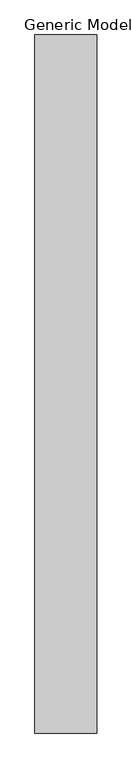
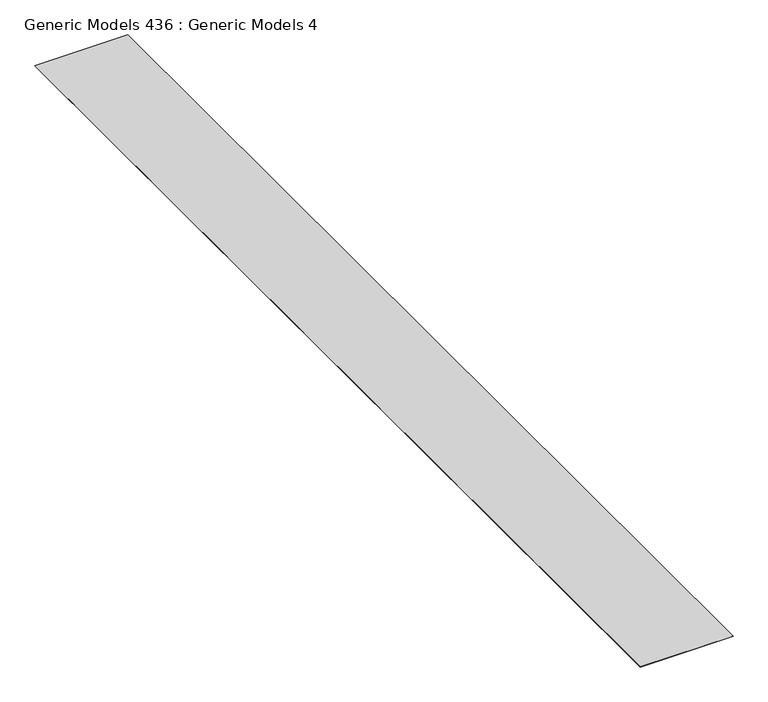
"""IFC4 building model written with IfcOpenShell, lengths in millimetres: proxy geometry, Generic Models 436 : Generic Models 4."""

from ifc_helpers import new_model, si_unit, frame, origin, place, context, project, spatial, polyline, outline, extrude, source, transform, mapped, element, save


def generic_models_436_generic_models_4_e7a1f224(model_context):
    return source(origin(), model_context, "Body", "SweptSolid", [
        extrude(outline(polyline([(9684.9758543, -5493.3230338), (8572.3263705, -5493.3230338), (8572.3263705, 7054.2769662), (9684.9758543, 7054.2769662), (9684.9758543, -5493.3230338)])), frame((0.0, 0.0, 123244.2139347), z_axis=(0.0, 0.0, 1.0), x_axis=(1.0, 0.0, 0.0)), (0.0, 0.0, 1.0), 1.5875),
    ])


if __name__ == "__main__":
    model = new_model("IFC4")
    model_context = context("Model", 3, world=origin())
    ifc_project = project(units=[si_unit("LENGTHUNIT", "METRE", prefix="MILLI")], contexts=[model_context])
    site = spatial("IfcSite", under=ifc_project)
    building = spatial("IfcBuilding", under=site)
    placement = place(None, origin())
    generic_models_436_generic_models_4_shape = generic_models_436_generic_models_4_e7a1f224(model_context)
    element("IfcBuildingElementProxy", 1, Name="Generic Models 436 : Generic Models 4", ObjectType="Generic Models 436 : Generic Models 4", at=placement, inside=building, context=model_context, shape_type="MappedRepresentation", body=[
        mapped(generic_models_436_generic_models_4_shape, transform((0.0, 0.0, 0.0), x_axis=(1.0, 0.0, 0.0), y_axis=(0.0, 1.0, 0.0), z_axis=(0.0, 0.0, 1.0))),
    ])
    save(model, "model.ifc")

# Revit data of these elements
# Element 1 (IfcBuildingElementProxy, "Generic Models 436 : Generic Models 4")
#   Materials on its faces: "_GEOTEXTILE FABRIC - TURN UP AT EDGES"
# Materials
#   "_GEOTEXTILE FABRIC - TURN UP AT EDGES": class "Generic", colour RGB 253 192 103, transparency 0, Cost = 0
